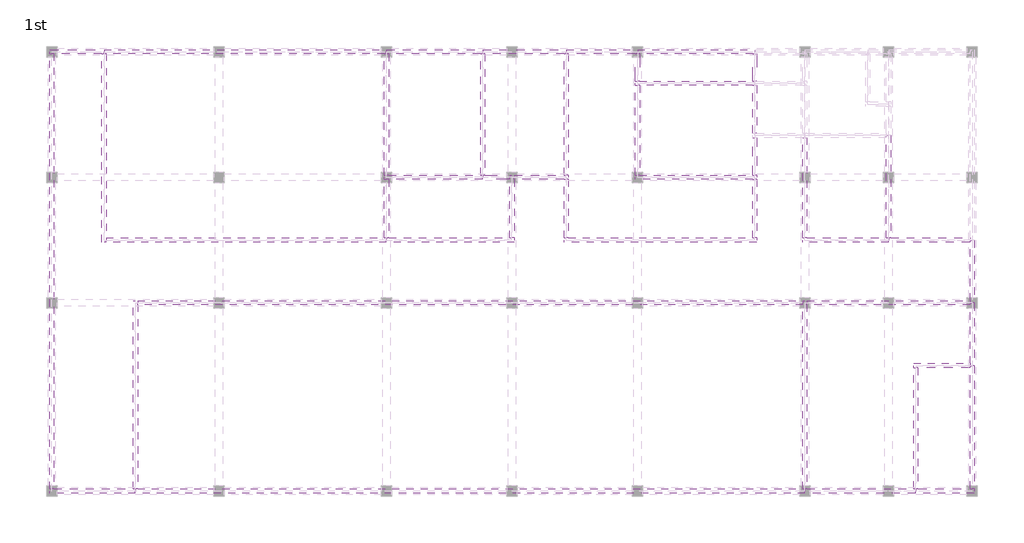
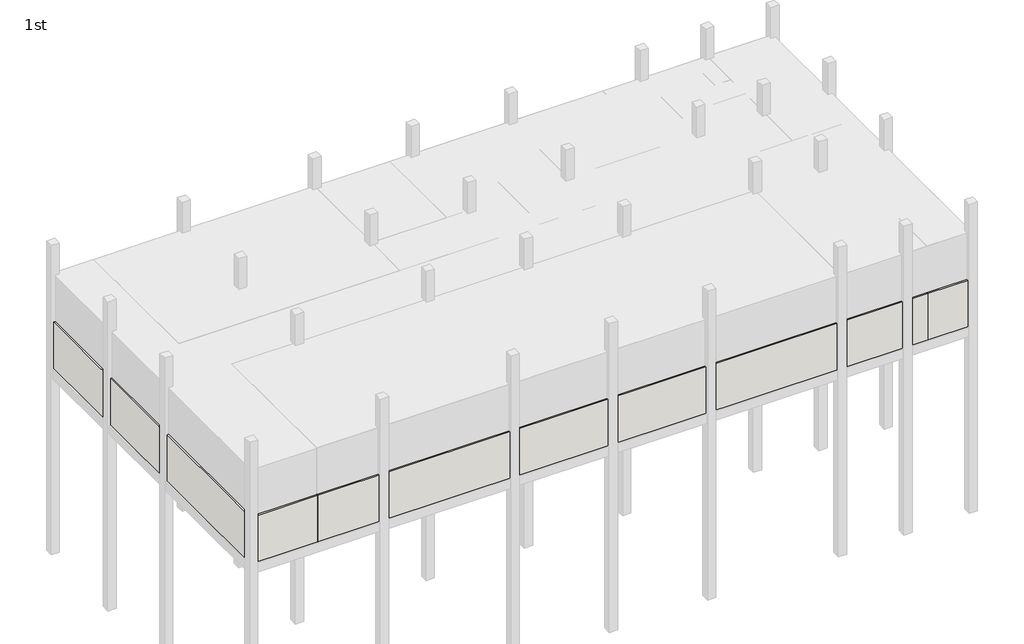
# One storey, part 1 of 3: 45 walls.
"""IFC4 building model written with IfcOpenShell, lengths in millimetres."""

from ifc_helpers import new_model, si_unit, frame, origin, place, context, project, spatial, polyline, outline, extrude, faceted_brep, element, save

model = new_model("IFC4")

# Units and contexts
model_context = context("Model", 3, world=origin())
ifc_project = project(units=[si_unit("LENGTHUNIT", "METRE", prefix="MILLI")], contexts=[model_context])

# Site, building, storey
site = spatial("IfcSite", under=ifc_project)
building = spatial("IfcBuilding", under=site)
storey = spatial("IfcBuildingStorey", under=building, Name="1st", Elevation=6000.0)

# Walls
placement = place(None, origin())
element("IfcWall", 1, ObjectType="WA111-Exterior RC Wall 200mm", at=placement, inside=storey, context=model_context, shape_type="Brep", body=[
    faceted_brep([(49459.6521483, 163823.8614395, 12000.0), (81459.6521483, 163823.8614395, 12000.0), (81459.6521483, 163823.8614395, 15000.0), (49459.6521483, 163823.8614395, 15000.0), (49459.6521483, 164023.8614395, 12000.0), (49459.6521483, 164023.8614395, 15000.0), (49559.6521483, 164023.8614395, 15000.0), (81359.6521483, 164023.8614395, 15000.0), (81459.6521483, 164023.8614395, 15000.0), (81459.6521483, 164023.8614395, 12000.0), (81359.6521483, 164023.8614395, 12000.0), (49559.6521483, 164023.8614395, 12000.0)], [[[0, 1, 2, 3]], [[4, 5, 6, 7, 8, 9, 10, 11]], [[1, 0, 4, 11, 10, 9]], [[2, 1, 9, 8]], [[3, 2, 8, 7, 6, 5]], [[0, 3, 5, 4]]]),
])
element("IfcWall", 2, ObjectType="WA111-Exterior RC Wall 200mm", at=placement, inside=storey, context=model_context, shape_type="Brep", body=[
    faceted_brep([(61459.6521483, 185023.8614395, 12000.0), (47959.6521483, 185023.8614395, 12000.0), (47959.6521483, 185023.8614395, 15000.0), (61459.6521483, 185023.8614395, 15000.0), (61459.6521483, 184823.8614395, 12000.0), (61459.6521483, 184823.8614395, 15000.0), (61359.6521483, 184823.8614395, 15000.0), (48059.6521483, 184823.8614395, 15000.0), (47959.6521483, 184823.8614395, 15000.0), (47959.6521483, 184823.8614395, 12000.0), (48059.6521483, 184823.8614395, 12000.0), (61359.6521483, 184823.8614395, 12000.0)], [[[0, 1, 2, 3]], [[4, 5, 6, 7, 8, 9, 10, 11]], [[1, 0, 4, 11, 10, 9]], [[2, 1, 9, 8]], [[3, 2, 8, 7, 6, 5]], [[0, 3, 5, 4]]]),
])
element("IfcWall", 3, ObjectType="WA111-Exterior RC Wall 200mm", at=placement, inside=storey, context=model_context, shape_type="Brep", body=[
    faceted_brep([(66059.6521483, 185023.8614395, 12000.0), (61459.6521483, 185023.8614395, 12000.0), (61459.6521483, 185023.8614395, 15000.0), (66059.6521483, 185023.8614395, 15000.0), (66059.6521483, 184823.8614395, 12000.0), (66059.6521483, 184823.8614395, 15000.0), (65959.6521483, 184823.8614395, 15000.0), (61559.6521483, 184823.8614395, 15000.0), (61459.6521483, 184823.8614395, 15000.0), (61459.6521483, 184823.8614395, 12000.0), (61559.6521483, 184823.8614395, 12000.0), (65959.6521483, 184823.8614395, 12000.0)], [[[0, 1, 2, 3]], [[4, 5, 6, 7, 8, 9, 10, 11]], [[1, 0, 4, 11, 10, 9]], [[2, 1, 9, 8]], [[3, 2, 8, 7, 6, 5]], [[0, 3, 5, 4]]]),
])
element("IfcWall", 4, ObjectType="WA111-Exterior RC Wall 200mm", at=placement, inside=storey, context=model_context, shape_type="Brep", body=[
    faceted_brep([(70059.6521483, 185023.8614395, 12000.0), (66059.6521483, 185023.8614395, 12000.0), (66059.6521483, 185023.8614395, 15000.0), (70059.6521483, 185023.8614395, 15000.0), (70059.6521483, 184823.8614395, 12000.0), (70059.6521483, 184823.8614395, 15000.0), (69959.6521483, 184823.8614395, 15000.0), (66159.6521483, 184823.8614395, 15000.0), (66059.6521483, 184823.8614395, 15000.0), (66059.6521483, 184823.8614395, 12000.0), (66159.6521483, 184823.8614395, 12000.0), (69959.6521483, 184823.8614395, 12000.0)], [[[0, 1, 2, 3]], [[4, 5, 6, 7, 8, 9, 10, 11]], [[1, 0, 4, 11, 10, 9]], [[2, 1, 9, 8]], [[3, 2, 8, 7, 6, 5]], [[0, 3, 5, 4]]]),
])
element("IfcWall", 5, ObjectType="WA111-Exterior RC Wall 200mm", at=placement, inside=storey, context=model_context, shape_type="Brep", body=[
    faceted_brep([(89559.6521483, 172923.8614395, 12000.0), (89559.6521483, 175923.8614395, 12000.0), (89559.6521483, 175923.8614395, 15000.0), (89559.6521483, 172923.8614395, 15000.0), (89359.6521483, 172923.8614395, 12000.0), (89359.6521483, 172923.8614395, 15000.0), (89359.6521483, 173023.8614395, 15000.0), (89359.6521483, 175823.8614395, 15000.0), (89359.6521483, 175923.8614395, 15000.0), (89359.6521483, 175923.8614395, 12000.0), (89359.6521483, 175823.8614395, 12000.0), (89359.6521483, 173023.8614395, 12000.0)], [[[0, 1, 2, 3]], [[4, 5, 6, 7, 8, 9, 10, 11]], [[1, 0, 4, 11, 10, 9]], [[2, 1, 9, 8]], [[3, 2, 8, 7, 6, 5]], [[0, 3, 5, 4]]]),
])
element("IfcWall", 6, ObjectType="WA111-Exterior RC Wall 200mm", at=placement, inside=storey, context=model_context, shape_type="Brep", body=[
    faceted_brep([(47959.6521483, 185023.8614395, 12000.0), (45359.6521483, 185023.8614395, 12000.0), (45359.6521483, 185023.8614395, 15000.0), (47959.6521483, 185023.8614395, 15000.0), (47959.6521483, 184823.8614395, 12000.0), (47959.6521483, 184823.8614395, 15000.0), (47859.6521483, 184823.8614395, 15000.0), (45559.6521483, 184823.8614395, 15000.0), (45359.6521483, 184823.8614395, 15000.0), (45359.6521483, 184823.8614395, 12000.0), (45559.6521483, 184823.8614395, 12000.0), (47859.6521483, 184823.8614395, 12000.0)], [[[0, 1, 2, 3]], [[4, 5, 6, 7, 8, 9, 10, 11]], [[1, 0, 4, 11, 10, 9]], [[3, 2, 8, 7, 6, 5]], [[0, 3, 5, 4]], [[2, 1, 9, 8]]]),
])
element("IfcWall", 7, ObjectType="WA111-Exterior RC Wall 200mm", at=placement, inside=storey, context=model_context, shape_type="SweptSolid", body=[
    extrude(outline(polyline([(45359.6521483, 164023.8614395), (45359.6521483, 184823.8614395), (45559.6521483, 184823.8614395), (45559.6521483, 164023.8614395), (45359.6521483, 164023.8614395)])), frame((0.0, 0.0, 12000.0), z_axis=(0.0, 0.0, 1.0), x_axis=(1.0, 0.0, 0.0)), (0.0, 0.0, 1.0), 3000.0),
])
element("IfcWall", 8, ObjectType="WA111-Exterior RC Wall 200mm", at=placement, inside=storey, context=model_context, shape_type="Brep", body=[
    faceted_brep([(45359.6521483, 163823.8614395, 12000.0), (49459.6521483, 163823.8614395, 12000.0), (49459.6521483, 163823.8614395, 15000.0), (45359.6521483, 163823.8614395, 15000.0), (45359.6521483, 164023.8614395, 12000.0), (45359.6521483, 164023.8614395, 15000.0), (45559.6521483, 164023.8614395, 15000.0), (49359.6521483, 164023.8614395, 15000.0), (49459.6521483, 164023.8614395, 15000.0), (49459.6521483, 164023.8614395, 12000.0), (49359.6521483, 164023.8614395, 12000.0), (45559.6521483, 164023.8614395, 12000.0)], [[[0, 1, 2, 3]], [[4, 5, 6, 7, 8, 9, 10, 11]], [[1, 0, 4, 11, 10, 9]], [[2, 1, 9, 8]], [[3, 2, 8, 7, 6, 5]], [[0, 3, 5, 4]]]),
])
element("IfcWall", 9, ObjectType="WA111-Exterior RC Wall 200mm", at=placement, inside=storey, context=model_context, shape_type="Brep", body=[
    faceted_brep([(79059.6521483, 185023.8614395, 12000.0), (73459.6521483, 185023.8614395, 12000.0), (73459.6521483, 185023.8614395, 15000.0), (79059.6521483, 185023.8614395, 15000.0), (79059.6521483, 184823.8614395, 12000.0), (79059.6521483, 184823.8614395, 15000.0), (78959.6521483, 184823.8614395, 15000.0), (73559.6521483, 184823.8614395, 15000.0), (73459.6521483, 184823.8614395, 15000.0), (73459.6521483, 184823.8614395, 12000.0), (73559.6521483, 184823.8614395, 12000.0), (78959.6521483, 184823.8614395, 12000.0)], [[[0, 1, 2, 3]], [[4, 5, 6, 7, 8, 9, 10, 11]], [[1, 0, 4, 11, 10, 9]], [[2, 1, 9, 8]], [[3, 2, 8, 7, 6, 5]], [[0, 3, 5, 4]]]),
])
element("IfcWall", 10, ObjectType="WA111-Exterior RC Wall 200mm", at=placement, inside=storey, context=model_context, shape_type="Brep", body=[
    faceted_brep([(73459.6521483, 185023.8614395, 12000.0), (70059.6521483, 185023.8614395, 12000.0), (70059.6521483, 185023.8614395, 15000.0), (73459.6521483, 185023.8614395, 15000.0), (73459.6521483, 184823.8614395, 12000.0), (73459.6521483, 184823.8614395, 15000.0), (73359.6521483, 184823.8614395, 15000.0), (70159.6521483, 184823.8614395, 15000.0), (70059.6521483, 184823.8614395, 15000.0), (70059.6521483, 184823.8614395, 12000.0), (70159.6521483, 184823.8614395, 12000.0), (73359.6521483, 184823.8614395, 12000.0)], [[[0, 1, 2, 3]], [[4, 5, 6, 7, 8, 9, 10, 11]], [[1, 0, 4, 11, 10, 9]], [[2, 1, 9, 8]], [[3, 2, 8, 7, 6, 5]], [[0, 3, 5, 4]]]),
])
element("IfcWall", 11, ObjectType="WA111-Exterior RC Wall 200mm", at=placement, inside=storey, context=model_context, shape_type="Brep", body=[
    faceted_brep([(81459.6521483, 163823.8614395, 12000.0), (86759.6521483, 163823.8614395, 12000.0), (86759.6521483, 163823.8614395, 15000.0), (81459.6521483, 163823.8614395, 15000.0), (81459.6521483, 164023.8614395, 12000.0), (81459.6521483, 164023.8614395, 15000.0), (81559.6521483, 164023.8614395, 15000.0), (86659.6521483, 164023.8614395, 15000.0), (86759.6521483, 164023.8614395, 15000.0), (86759.6521483, 164023.8614395, 12000.0), (86659.6521483, 164023.8614395, 12000.0), (81559.6521483, 164023.8614395, 12000.0)], [[[0, 1, 2, 3]], [[4, 5, 6, 7, 8, 9, 10, 11]], [[1, 0, 4, 11, 10, 9]], [[2, 1, 9, 8]], [[3, 2, 8, 7, 6, 5]], [[0, 3, 5, 4]]]),
])
element("IfcWall", 12, ObjectType="WA111-Exterior RC Wall 200mm", at=placement, inside=storey, context=model_context, shape_type="Brep", body=[
    faceted_brep([(89559.6521483, 169923.8614395, 12000.0), (89559.6521483, 172923.8614395, 12000.0), (89559.6521483, 172923.8614395, 15000.0), (89559.6521483, 169923.8614395, 15000.0), (89359.6521483, 169923.8614395, 12000.0), (89359.6521483, 169923.8614395, 15000.0), (89359.6521483, 170023.8614395, 15000.0), (89359.6521483, 172823.8614395, 15000.0), (89359.6521483, 172923.8614395, 15000.0), (89359.6521483, 172923.8614395, 12000.0), (89359.6521483, 172823.8614395, 12000.0), (89359.6521483, 170023.8614395, 12000.0)], [[[0, 1, 2, 3]], [[4, 5, 6, 7, 8, 9, 10, 11]], [[1, 0, 4, 11, 10, 9]], [[2, 1, 9, 8]], [[3, 2, 8, 7, 6, 5]], [[0, 3, 5, 4]]]),
])
element("IfcWall", 13, ObjectType="WA111-Exterior RC Wall 200mm", at=placement, inside=storey, context=model_context, shape_type="Brep", body=[
    faceted_brep([(89559.6521483, 164023.8614395, 12000.0), (89559.6521483, 169923.8614395, 12000.0), (89559.6521483, 169923.8614395, 15000.0), (89559.6521483, 164023.8614395, 15000.0), (89359.6521483, 164023.8614395, 12000.0), (89359.6521483, 164023.8614395, 15000.0), (89359.6521483, 169823.8614395, 15000.0), (89359.6521483, 169923.8614395, 15000.0), (89359.6521483, 169923.8614395, 12000.0), (89359.6521483, 169823.8614395, 12000.0)], [[[0, 1, 2, 3]], [[4, 5, 6, 7, 8, 9]], [[1, 0, 4, 9, 8]], [[2, 1, 8, 7]], [[3, 2, 7, 6, 5]], [[0, 3, 5, 4]]]),
])
element("IfcWall", 14, ObjectType="WA111-Exterior RC Wall 200mm", at=placement, inside=storey, context=model_context, shape_type="Brep", body=[
    faceted_brep([(86759.6521483, 163823.8614395, 12000.0), (89559.6521483, 163823.8614395, 12000.0), (89559.6521483, 163823.8614395, 15000.0), (86759.6521483, 163823.8614395, 15000.0), (86759.6521483, 164023.8614395, 12000.0), (86759.6521483, 164023.8614395, 15000.0), (86859.6521483, 164023.8614395, 15000.0), (89359.6521483, 164023.8614395, 15000.0), (89559.6521483, 164023.8614395, 15000.0), (89559.6521483, 164023.8614395, 12000.0), (89359.6521483, 164023.8614395, 12000.0), (86859.6521483, 164023.8614395, 12000.0)], [[[0, 1, 2, 3]], [[4, 5, 6, 7, 8, 9, 10, 11]], [[1, 0, 4, 11, 10, 9]], [[3, 2, 8, 7, 6, 5]], [[0, 3, 5, 4]], [[2, 1, 9, 8]]]),
])
element("IfcWall", 15, ObjectType="WA121-Interior RC Wall 200mm", at=placement, inside=storey, context=model_context, shape_type="SweptSolid", body=[
    extrude(outline(polyline([(49559.6521483, 173023.8614395), (81359.6521483, 173023.8614395), (81359.6521483, 172823.8614395), (49559.6521483, 172823.8614395), (49559.6521483, 173023.8614395)])), frame((0.0, 0.0, 12000.0), z_axis=(0.0, 0.0, 1.0), x_axis=(1.0, 0.0, 0.0)), (0.0, 0.0, 1.0), 3000.0),
])
element("IfcWall", 16, ObjectType="WA121-Interior RC Wall 200mm", at=placement, inside=storey, context=model_context, shape_type="Brep", body=[
    faceted_brep([(49359.6521483, 173023.8614395, 12000.0), (49359.6521483, 164023.8614395, 12000.0), (49359.6521483, 164023.8614395, 15000.0), (49359.6521483, 173023.8614395, 15000.0), (49559.6521483, 173023.8614395, 12000.0), (49559.6521483, 173023.8614395, 15000.0), (49559.6521483, 172823.8614395, 15000.0), (49559.6521483, 164023.8614395, 15000.0), (49559.6521483, 164023.8614395, 12000.0), (49559.6521483, 172823.8614395, 12000.0), (49459.6521483, 164023.8614395, 12000.0), (49459.6521483, 164023.8614395, 15000.0)], [[[0, 1, 2, 3]], [[4, 5, 6, 7, 8, 9]], [[1, 0, 4, 9, 8, 10]], [[3, 2, 11, 7, 6, 5]], [[0, 3, 5, 4]], [[2, 1, 10, 8, 7, 11]]]),
])
element("IfcWall", 17, ObjectType="WA121-Interior RC Wall 200mm", at=placement, inside=storey, context=model_context, shape_type="Brep", body=[
    faceted_brep([(81559.6521483, 164023.8614395, 12000.0), (81559.6521483, 172823.8614395, 12000.0), (81559.6521483, 173023.8614395, 12000.0), (81559.6521483, 173023.8614395, 15000.0), (81559.6521483, 172823.8614395, 15000.0), (81559.6521483, 164023.8614395, 15000.0), (81359.6521483, 164023.8614395, 12000.0), (81359.6521483, 164023.8614395, 15000.0), (81359.6521483, 172823.8614395, 15000.0), (81359.6521483, 173023.8614395, 15000.0), (81359.6521483, 173023.8614395, 12000.0), (81359.6521483, 172823.8614395, 12000.0), (81459.6521483, 164023.8614395, 12000.0), (81459.6521483, 164023.8614395, 15000.0)], [[[0, 1, 2, 3, 4, 5]], [[6, 7, 8, 9, 10, 11]], [[2, 1, 0, 12, 6, 11, 10]], [[5, 4, 3, 9, 8, 7, 13]], [[3, 2, 10, 9]], [[0, 5, 13, 7, 6, 12]]]),
])
element("IfcWall", 18, ObjectType="WA121-Interior RC Wall 200mm", at=placement, inside=storey, context=model_context, shape_type="Brep", body=[
    faceted_brep([(47859.6521483, 184823.8614395, 12000.0), (47859.6521483, 175823.8614395, 12000.0), (47859.6521483, 175823.8614395, 15000.0), (47859.6521483, 184823.8614395, 15000.0), (48059.6521483, 184823.8614395, 12000.0), (48059.6521483, 184823.8614395, 15000.0), (48059.6521483, 176023.8614395, 15000.0), (48059.6521483, 175823.8614395, 15000.0), (48059.6521483, 175823.8614395, 12000.0), (48059.6521483, 176023.8614395, 12000.0), (47959.6521483, 184823.8614395, 12000.0), (47959.6521483, 184823.8614395, 15000.0)], [[[0, 1, 2, 3]], [[4, 5, 6, 7, 8, 9]], [[1, 0, 10, 4, 9, 8]], [[3, 2, 7, 6, 5, 11]], [[0, 3, 11, 5, 4, 10]], [[2, 1, 8, 7]]]),
])
element("IfcWall", 19, ObjectType="WA121-Interior RC Wall 200mm", at=placement, inside=storey, context=model_context, shape_type="Brep", body=[
    faceted_brep([(48059.6521483, 175823.8614395, 12000.0), (61459.6521483, 175823.8614395, 12000.0), (61459.6521483, 175823.8614395, 15000.0), (48059.6521483, 175823.8614395, 15000.0), (48059.6521483, 176023.8614395, 12000.0), (48059.6521483, 176023.8614395, 15000.0), (61359.6521483, 176023.8614395, 15000.0), (61459.6521483, 176023.8614395, 15000.0), (61459.6521483, 176023.8614395, 12000.0), (61359.6521483, 176023.8614395, 12000.0)], [[[0, 1, 2, 3]], [[4, 5, 6, 7, 8, 9]], [[1, 0, 4, 9, 8]], [[2, 1, 8, 7]], [[3, 2, 7, 6, 5]], [[0, 3, 5, 4]]]),
])
element("IfcWall", 20, ObjectType="WA121-Interior RC Wall 200mm", at=placement, inside=storey, context=model_context, shape_type="Brep", body=[
    faceted_brep([(61559.6521483, 176023.8614395, 12000.0), (61559.6521483, 178823.8614395, 12000.0), (61559.6521483, 178823.8614395, 15000.0), (61559.6521483, 176023.8614395, 15000.0), (61359.6521483, 176023.8614395, 12000.0), (61359.6521483, 176023.8614395, 15000.0), (61359.6521483, 178823.8614395, 15000.0), (61359.6521483, 178823.8614395, 12000.0), (61459.6521483, 176023.8614395, 12000.0), (61459.6521483, 176023.8614395, 15000.0)], [[[0, 1, 2, 3]], [[4, 5, 6, 7]], [[1, 0, 8, 4, 7]], [[3, 2, 6, 5, 9]], [[0, 3, 9, 5, 4, 8]], [[2, 1, 7, 6]]]),
])
element("IfcWall", 21, ObjectType="WA121-Interior RC Wall 200mm", at=placement, inside=storey, context=model_context, shape_type="Brep", body=[
    faceted_brep([(61559.6521483, 179023.8614395, 12000.0), (61559.6521483, 184823.8614395, 12000.0), (61559.6521483, 184823.8614395, 15000.0), (61559.6521483, 179023.8614395, 15000.0), (61359.6521483, 179023.8614395, 12000.0), (61359.6521483, 179023.8614395, 15000.0), (61359.6521483, 184823.8614395, 15000.0), (61359.6521483, 184823.8614395, 12000.0), (61459.6521483, 184823.8614395, 12000.0), (61459.6521483, 184823.8614395, 15000.0)], [[[0, 1, 2, 3]], [[4, 5, 6, 7]], [[1, 0, 4, 7, 8]], [[3, 2, 9, 6, 5]], [[2, 1, 8, 7, 6, 9]], [[0, 3, 5, 4]]]),
])
element("IfcWall", 22, ObjectType="WA121-Interior RC Wall 200mm", at=placement, inside=storey, context=model_context, shape_type="Brep", body=[
    faceted_brep([(61359.6521483, 178823.8614395, 12000.0), (61559.6521483, 178823.8614395, 12000.0), (66059.6521483, 178823.8614395, 12000.0), (66059.6521483, 178823.8614395, 15000.0), (61559.6521483, 178823.8614395, 15000.0), (61359.6521483, 178823.8614395, 15000.0), (61359.6521483, 179023.8614395, 12000.0), (61359.6521483, 179023.8614395, 15000.0), (61559.6521483, 179023.8614395, 15000.0), (65959.6521483, 179023.8614395, 15000.0), (66059.6521483, 179023.8614395, 15000.0), (66059.6521483, 179023.8614395, 12000.0), (65959.6521483, 179023.8614395, 12000.0), (61559.6521483, 179023.8614395, 12000.0)], [[[0, 1, 2, 3, 4, 5]], [[6, 7, 8, 9, 10, 11, 12, 13]], [[2, 1, 0, 6, 13, 12, 11]], [[3, 2, 11, 10]], [[5, 4, 3, 10, 9, 8, 7]], [[0, 5, 7, 6]]]),
])
element("IfcWall", 23, ObjectType="WA121-Interior RC Wall 200mm", at=placement, inside=storey, context=model_context, shape_type="Brep", body=[
    faceted_brep([(66159.6521483, 179023.8614395, 12000.0), (66159.6521483, 184823.8614395, 12000.0), (66159.6521483, 184823.8614395, 15000.0), (66159.6521483, 179023.8614395, 15000.0), (65959.6521483, 179023.8614395, 12000.0), (65959.6521483, 179023.8614395, 15000.0), (65959.6521483, 184823.8614395, 15000.0), (65959.6521483, 184823.8614395, 12000.0), (66059.6521483, 179023.8614395, 12000.0), (66059.6521483, 184823.8614395, 12000.0), (66059.6521483, 184823.8614395, 15000.0), (66059.6521483, 179023.8614395, 15000.0)], [[[0, 1, 2, 3]], [[4, 5, 6, 7]], [[1, 0, 8, 4, 7, 9]], [[3, 2, 10, 6, 5, 11]], [[2, 1, 9, 7, 6, 10]], [[0, 3, 11, 5, 4, 8]]]),
])
element("IfcWall", 24, ObjectType="WA121-Interior RC Wall 200mm", at=placement, inside=storey, context=model_context, shape_type="Brep", body=[
    faceted_brep([(81359.6521483, 180823.8614395, 12000.0), (81359.6521483, 176023.8614395, 12000.0), (81359.6521483, 176023.8614395, 15000.0), (81359.6521483, 180823.8614395, 15000.0), (81559.6521483, 180823.8614395, 12000.0), (81559.6521483, 180823.8614395, 15000.0), (81559.6521483, 176023.8614395, 15000.0), (81559.6521483, 176023.8614395, 12000.0), (81459.6521483, 180823.8614395, 12000.0), (81459.6521483, 180823.8614395, 15000.0)], [[[0, 1, 2, 3]], [[4, 5, 6, 7]], [[1, 0, 8, 4, 7]], [[3, 2, 6, 5, 9]], [[0, 3, 9, 5, 4, 8]], [[2, 1, 7, 6]]]),
])
element("IfcWall", 25, ObjectType="WA121-Interior RC Wall 200mm", at=placement, inside=storey, context=model_context, shape_type="Brep", body=[
    faceted_brep([(81359.6521483, 175823.8614395, 12000.0), (85459.6521483, 175823.8614395, 12000.0), (85459.6521483, 175823.8614395, 15000.0), (81359.6521483, 175823.8614395, 15000.0), (81359.6521483, 176023.8614395, 12000.0), (81359.6521483, 176023.8614395, 15000.0), (81559.6521483, 176023.8614395, 15000.0), (85359.6521483, 176023.8614395, 15000.0), (85459.6521483, 176023.8614395, 15000.0), (85459.6521483, 176023.8614395, 12000.0), (85359.6521483, 176023.8614395, 12000.0), (81559.6521483, 176023.8614395, 12000.0)], [[[0, 1, 2, 3]], [[4, 5, 6, 7, 8, 9, 10, 11]], [[1, 0, 4, 11, 10, 9]], [[2, 1, 9, 8]], [[3, 2, 8, 7, 6, 5]], [[0, 3, 5, 4]]]),
])
element("IfcWall", 26, ObjectType="WA121-Interior RC Wall 200mm", at=placement, inside=storey, context=model_context, shape_type="Brep", body=[
    faceted_brep([(85559.6521483, 176023.8614395, 12000.0), (85559.6521483, 180923.8614395, 12000.0), (85559.6521483, 180923.8614395, 15000.0), (85559.6521483, 176023.8614395, 15000.0), (85359.6521483, 176023.8614395, 12000.0), (85359.6521483, 176023.8614395, 15000.0), (85359.6521483, 180823.8614395, 15000.0), (85359.6521483, 180923.8614395, 15000.0), (85359.6521483, 180923.8614395, 12000.0), (85359.6521483, 180823.8614395, 12000.0), (85459.6521483, 176023.8614395, 12000.0), (85459.6521483, 176023.8614395, 15000.0)], [[[0, 1, 2, 3]], [[4, 5, 6, 7, 8, 9]], [[1, 0, 10, 4, 9, 8]], [[2, 1, 8, 7]], [[3, 2, 7, 6, 5, 11]], [[0, 3, 11, 5, 4, 10]]]),
])
element("IfcWall", 27, ObjectType="WA121-Interior RC Wall 200mm", at=placement, inside=storey, context=model_context, shape_type="Brep", body=[
    faceted_brep([(85459.6521483, 175823.8614395, 12000.0), (89359.6521483, 175823.8614395, 12000.0), (89359.6521483, 175823.8614395, 15000.0), (85459.6521483, 175823.8614395, 15000.0), (85459.6521483, 176023.8614395, 12000.0), (85459.6521483, 176023.8614395, 15000.0), (85559.6521483, 176023.8614395, 15000.0), (89359.6521483, 176023.8614395, 15000.0), (89359.6521483, 176023.8614395, 12000.0), (85559.6521483, 176023.8614395, 12000.0), (89359.6521483, 175923.8614395, 12000.0), (89359.6521483, 175923.8614395, 15000.0)], [[[0, 1, 2, 3]], [[4, 5, 6, 7, 8, 9]], [[1, 0, 4, 9, 8, 10]], [[3, 2, 11, 7, 6, 5]], [[0, 3, 5, 4]], [[2, 1, 10, 8, 7, 11]]]),
])
element("IfcWall", 28, ObjectType="WA121-Interior RC Wall 200mm", at=placement, inside=storey, context=model_context, shape_type="Brep", body=[
    faceted_brep([(66059.6521483, 178823.8614395, 12000.0), (67359.6521483, 178823.8614395, 12000.0), (67359.6521483, 178823.8614395, 15000.0), (66059.6521483, 178823.8614395, 15000.0), (66059.6521483, 179023.8614395, 12000.0), (66059.6521483, 179023.8614395, 15000.0), (66159.6521483, 179023.8614395, 15000.0), (67359.6521483, 179023.8614395, 15000.0), (67359.6521483, 179023.8614395, 12000.0), (66159.6521483, 179023.8614395, 12000.0)], [[[0, 1, 2, 3]], [[4, 5, 6, 7, 8, 9]], [[1, 0, 4, 9, 8]], [[3, 2, 7, 6, 5]], [[0, 3, 5, 4]], [[2, 1, 8, 7]]]),
])
element("IfcWall", 29, ObjectType="WA121-Interior RC Wall 200mm", at=placement, inside=storey, context=model_context, shape_type="Brep", body=[
    faceted_brep([(67559.6521483, 178823.8614395, 12000.0), (69959.6521483, 178823.8614395, 12000.0), (70159.6521483, 178823.8614395, 12000.0), (70159.6521483, 178823.8614395, 15000.0), (69959.6521483, 178823.8614395, 15000.0), (67559.6521483, 178823.8614395, 15000.0), (67559.6521483, 179023.8614395, 12000.0), (67559.6521483, 179023.8614395, 15000.0), (69959.6521483, 179023.8614395, 15000.0), (70159.6521483, 179023.8614395, 15000.0), (70159.6521483, 179023.8614395, 12000.0), (69959.6521483, 179023.8614395, 12000.0)], [[[0, 1, 2, 3, 4, 5]], [[6, 7, 8, 9, 10, 11]], [[2, 1, 0, 6, 11, 10]], [[5, 4, 3, 9, 8, 7]], [[3, 2, 10, 9]], [[0, 5, 7, 6]]]),
])
element("IfcWall", 30, ObjectType="WA121-Interior RC Wall 200mm", at=placement, inside=storey, context=model_context, shape_type="Brep", body=[
    faceted_brep([(70159.6521483, 179023.8614395, 12000.0), (70159.6521483, 184823.8614395, 12000.0), (70159.6521483, 184823.8614395, 15000.0), (70159.6521483, 179023.8614395, 15000.0), (69959.6521483, 179023.8614395, 12000.0), (69959.6521483, 179023.8614395, 15000.0), (69959.6521483, 184823.8614395, 15000.0), (69959.6521483, 184823.8614395, 12000.0), (70059.6521483, 184823.8614395, 12000.0), (70059.6521483, 184823.8614395, 15000.0)], [[[0, 1, 2, 3]], [[4, 5, 6, 7]], [[1, 0, 4, 7, 8]], [[3, 2, 9, 6, 5]], [[2, 1, 8, 7, 6, 9]], [[0, 3, 5, 4]]]),
])
element("IfcWall", 31, ObjectType="WA121-Interior RC Wall 200mm", at=placement, inside=storey, context=model_context, shape_type="Brep", body=[
    faceted_brep([(61459.6521483, 175823.8614395, 12000.0), (67559.6521483, 175823.8614395, 12000.0), (67559.6521483, 175823.8614395, 15000.0), (61459.6521483, 175823.8614395, 15000.0), (61459.6521483, 176023.8614395, 12000.0), (61459.6521483, 176023.8614395, 15000.0), (61559.6521483, 176023.8614395, 15000.0), (67359.6521483, 176023.8614395, 15000.0), (67559.6521483, 176023.8614395, 15000.0), (67559.6521483, 176023.8614395, 12000.0), (67359.6521483, 176023.8614395, 12000.0), (61559.6521483, 176023.8614395, 12000.0)], [[[0, 1, 2, 3]], [[4, 5, 6, 7, 8, 9, 10, 11]], [[1, 0, 4, 11, 10, 9]], [[3, 2, 8, 7, 6, 5]], [[0, 3, 5, 4]], [[2, 1, 9, 8]]]),
])
element("IfcWall", 32, ObjectType="WA121-Interior RC Wall 200mm", at=placement, inside=storey, context=model_context, shape_type="Brep", body=[
    faceted_brep([(67559.6521483, 176023.8614395, 12000.0), (67559.6521483, 178823.8614395, 12000.0), (67559.6521483, 179023.8614395, 12000.0), (67559.6521483, 179023.8614395, 15000.0), (67559.6521483, 178823.8614395, 15000.0), (67559.6521483, 176023.8614395, 15000.0), (67359.6521483, 176023.8614395, 12000.0), (67359.6521483, 176023.8614395, 15000.0), (67359.6521483, 178823.8614395, 15000.0), (67359.6521483, 179023.8614395, 15000.0), (67359.6521483, 179023.8614395, 12000.0), (67359.6521483, 178823.8614395, 12000.0)], [[[0, 1, 2, 3, 4, 5]], [[6, 7, 8, 9, 10, 11]], [[2, 1, 0, 6, 11, 10]], [[5, 4, 3, 9, 8, 7]], [[3, 2, 10, 9]], [[0, 5, 7, 6]]]),
])
element("IfcWall", 33, ObjectType="WA121-Interior RC Wall 200mm", at=placement, inside=storey, context=model_context, shape_type="Brep", body=[
    faceted_brep([(78959.6521483, 184823.8614395, 12000.0), (78959.6521483, 183523.8614395, 12000.0), (78959.6521483, 183523.8614395, 15000.0), (78959.6521483, 184823.8614395, 15000.0), (79159.6521483, 184823.8614395, 12000.0), (79159.6521483, 184823.8614395, 15000.0), (79159.6521483, 183523.8614395, 15000.0), (79159.6521483, 183523.8614395, 12000.0), (79059.6521483, 184823.8614395, 12000.0), (79059.6521483, 183523.8614395, 12000.0), (79059.6521483, 183523.8614395, 15000.0), (79059.6521483, 184823.8614395, 15000.0)], [[[0, 1, 2, 3]], [[4, 5, 6, 7]], [[1, 0, 8, 4, 7, 9]], [[3, 2, 10, 6, 5, 11]], [[0, 3, 11, 5, 4, 8]], [[2, 1, 9, 7, 6, 10]]]),
])
element("IfcWall", 34, ObjectType="WA121-Interior RC Wall 200mm", at=placement, inside=storey, context=model_context, shape_type="Brep", body=[
    faceted_brep([(81559.6521483, 172823.8614395, 12000.0), (89359.6521483, 172823.8614395, 12000.0), (89359.6521483, 172823.8614395, 15000.0), (81559.6521483, 172823.8614395, 15000.0), (81559.6521483, 173023.8614395, 12000.0), (81559.6521483, 173023.8614395, 15000.0), (89359.6521483, 173023.8614395, 15000.0), (89359.6521483, 173023.8614395, 12000.0), (89359.6521483, 172923.8614395, 12000.0), (89359.6521483, 172923.8614395, 15000.0)], [[[0, 1, 2, 3]], [[4, 5, 6, 7]], [[1, 0, 4, 7, 8]], [[3, 2, 9, 6, 5]], [[0, 3, 5, 4]], [[2, 1, 8, 7, 6, 9]]]),
])
element("IfcWall", 35, ObjectType="WA121-Interior RC Wall 200mm", at=placement, inside=storey, context=model_context, shape_type="SweptSolid", body=[
    extrude(outline(polyline([(78959.6521483, 179023.8614395), (78959.6521483, 180823.8614395), (79159.6521483, 180823.8614395), (79159.6521483, 179023.8614395), (78959.6521483, 179023.8614395)])), frame((0.0, 0.0, 12000.0), z_axis=(0.0, 0.0, 1.0), x_axis=(1.0, 0.0, 0.0)), (0.0, 0.0, 1.0), 3000.0),
])
element("IfcWall", 36, ObjectType="WA121-Interior RC Wall 200mm", at=placement, inside=storey, context=model_context, shape_type="SweptSolid", body=[
    extrude(outline(polyline([(78959.6521483, 176023.8614395), (78959.6521483, 178823.8614395), (79159.6521483, 178823.8614395), (79159.6521483, 176023.8614395), (78959.6521483, 176023.8614395)])), frame((0.0, 0.0, 12000.0), z_axis=(0.0, 0.0, 1.0), x_axis=(1.0, 0.0, 0.0)), (0.0, 0.0, 1.0), 3000.0),
])
element("IfcWall", 37, ObjectType="WA121-Interior RC Wall 200mm", at=placement, inside=storey, context=model_context, shape_type="Brep", body=[
    faceted_brep([(79159.6521483, 176023.8614395, 12000.0), (78959.6521483, 176023.8614395, 12000.0), (70159.6521483, 176023.8614395, 12000.0), (69959.6521483, 176023.8614395, 12000.0), (69959.6521483, 176023.8614395, 15000.0), (70159.6521483, 176023.8614395, 15000.0), (78959.6521483, 176023.8614395, 15000.0), (79159.6521483, 176023.8614395, 15000.0), (79159.6521483, 175823.8614395, 12000.0), (79159.6521483, 175823.8614395, 15000.0), (69959.6521483, 175823.8614395, 15000.0), (69959.6521483, 175823.8614395, 12000.0)], [[[0, 1, 2, 3, 4, 5, 6, 7]], [[8, 9, 10, 11]], [[3, 2, 1, 0, 8, 11]], [[7, 6, 5, 4, 10, 9]], [[0, 7, 9, 8]], [[4, 3, 11, 10]]]),
])
element("IfcWall", 38, ObjectType="WA121-Interior RC Wall 200mm", at=placement, inside=storey, context=model_context, shape_type="SweptSolid", body=[
    extrude(outline(polyline([(70159.6521483, 178823.8614395), (70159.6521483, 176023.8614395), (69959.6521483, 176023.8614395), (69959.6521483, 178823.8614395), (70159.6521483, 178823.8614395)])), frame((0.0, 0.0, 12000.0), z_axis=(0.0, 0.0, 1.0), x_axis=(1.0, 0.0, 0.0)), (0.0, 0.0, 1.0), 3000.0),
])
element("IfcWall", 39, ObjectType="WA121-Interior RC Wall 200mm", at=placement, inside=storey, context=model_context, shape_type="Brep", body=[
    faceted_brep([(78959.6521483, 183323.8614395, 12000.0), (78959.6521483, 181023.8614395, 12000.0), (78959.6521483, 181023.8614395, 15000.0), (78959.6521483, 183323.8614395, 15000.0), (79159.6521483, 183323.8614395, 12000.0), (79159.6521483, 183323.8614395, 15000.0), (79159.6521483, 181023.8614395, 15000.0), (79159.6521483, 181023.8614395, 12000.0), (79059.6521483, 183323.8614395, 12000.0), (79059.6521483, 183323.8614395, 15000.0)], [[[0, 1, 2, 3]], [[4, 5, 6, 7]], [[1, 0, 8, 4, 7]], [[3, 2, 6, 5, 9]], [[0, 3, 9, 5, 4, 8]], [[2, 1, 7, 6]]]),
])
element("IfcWall", 40, ObjectType="WA121-Interior RC Wall 200mm", at=placement, inside=storey, context=model_context, shape_type="Brep", body=[
    faceted_brep([(73359.6521483, 184823.8614395, 12000.0), (73359.6521483, 183523.8614395, 12000.0), (73359.6521483, 183523.8614395, 15000.0), (73359.6521483, 184823.8614395, 15000.0), (73559.6521483, 184823.8614395, 12000.0), (73559.6521483, 184823.8614395, 15000.0), (73559.6521483, 183523.8614395, 15000.0), (73559.6521483, 183523.8614395, 12000.0), (73459.6521483, 184823.8614395, 12000.0), (73459.6521483, 184823.8614395, 15000.0)], [[[0, 1, 2, 3]], [[4, 5, 6, 7]], [[1, 0, 8, 4, 7]], [[3, 2, 6, 5, 9]], [[0, 3, 9, 5, 4, 8]], [[2, 1, 7, 6]]]),
])
element("IfcWall", 41, ObjectType="WA121-Interior RC Wall 200mm", at=placement, inside=storey, context=model_context, shape_type="Brep", body=[
    faceted_brep([(73359.6521483, 183323.8614395, 12000.0), (73559.6521483, 183323.8614395, 12000.0), (78959.6521483, 183323.8614395, 12000.0), (79059.6521483, 183323.8614395, 12000.0), (79059.6521483, 183323.8614395, 15000.0), (78959.6521483, 183323.8614395, 15000.0), (73559.6521483, 183323.8614395, 15000.0), (73359.6521483, 183323.8614395, 15000.0), (73359.6521483, 183523.8614395, 12000.0), (73359.6521483, 183523.8614395, 15000.0), (73559.6521483, 183523.8614395, 15000.0), (78959.6521483, 183523.8614395, 15000.0), (79059.6521483, 183523.8614395, 15000.0), (79059.6521483, 183523.8614395, 12000.0), (78959.6521483, 183523.8614395, 12000.0), (73559.6521483, 183523.8614395, 12000.0)], [[[0, 1, 2, 3, 4, 5, 6, 7]], [[8, 9, 10, 11, 12, 13, 14, 15]], [[3, 2, 1, 0, 8, 15, 14, 13]], [[4, 3, 13, 12]], [[7, 6, 5, 4, 12, 11, 10, 9]], [[0, 7, 9, 8]]]),
])
element("IfcWall", 42, ObjectType="WA121-Interior RC Wall 200mm", at=placement, inside=storey, context=model_context, shape_type="Brep", body=[
    faceted_brep([(79159.6521483, 179023.8614395, 12000.0), (78959.6521483, 179023.8614395, 12000.0), (73559.6521483, 179023.8614395, 12000.0), (73359.6521483, 179023.8614395, 12000.0), (73359.6521483, 179023.8614395, 15000.0), (73559.6521483, 179023.8614395, 15000.0), (78959.6521483, 179023.8614395, 15000.0), (79159.6521483, 179023.8614395, 15000.0), (79159.6521483, 178823.8614395, 12000.0), (79159.6521483, 178823.8614395, 15000.0), (78959.6521483, 178823.8614395, 15000.0), (73359.6521483, 178823.8614395, 15000.0), (73359.6521483, 178823.8614395, 12000.0), (78959.6521483, 178823.8614395, 12000.0)], [[[0, 1, 2, 3, 4, 5, 6, 7]], [[8, 9, 10, 11, 12, 13]], [[3, 2, 1, 0, 8, 13, 12]], [[7, 6, 5, 4, 11, 10, 9]], [[0, 7, 9, 8]], [[4, 3, 12, 11]]]),
])
element("IfcWall", 43, ObjectType="WA121-Interior RC Wall 200mm", at=placement, inside=storey, context=model_context, shape_type="SweptSolid", body=[
    extrude(outline(polyline([(73559.6521483, 183323.8614395), (73559.6521483, 179023.8614395), (73359.6521483, 179023.8614395), (73359.6521483, 183323.8614395), (73559.6521483, 183323.8614395)])), frame((0.0, 0.0, 12000.0), z_axis=(0.0, 0.0, 1.0), x_axis=(1.0, 0.0, 0.0)), (0.0, 0.0, 1.0), 3000.0),
])
element("IfcWall", 44, ObjectType="WA121-Interior RC Wall 200mm", at=placement, inside=storey, context=model_context, shape_type="Brep", body=[
    faceted_brep([(86859.6521483, 164023.8614395, 12000.0), (86859.6521483, 169823.8614395, 12000.0), (86859.6521483, 169823.8614395, 15000.0), (86859.6521483, 164023.8614395, 15000.0), (86659.6521483, 164023.8614395, 12000.0), (86659.6521483, 164023.8614395, 15000.0), (86659.6521483, 169823.8614395, 15000.0), (86659.6521483, 169823.8614395, 12000.0), (86759.6521483, 164023.8614395, 12000.0), (86759.6521483, 164023.8614395, 15000.0)], [[[0, 1, 2, 3]], [[4, 5, 6, 7]], [[1, 0, 8, 4, 7]], [[3, 2, 6, 5, 9]], [[2, 1, 7, 6]], [[0, 3, 9, 5, 4, 8]]]),
])
element("IfcWall", 45, ObjectType="WA121-Interior RC Wall 200mm", at=placement, inside=storey, context=model_context, shape_type="Brep", body=[
    faceted_brep([(86659.6521483, 169823.8614395, 12000.0), (86859.6521483, 169823.8614395, 12000.0), (89359.6521483, 169823.8614395, 12000.0), (89359.6521483, 169823.8614395, 15000.0), (86859.6521483, 169823.8614395, 15000.0), (86659.6521483, 169823.8614395, 15000.0), (86659.6521483, 170023.8614395, 12000.0), (86659.6521483, 170023.8614395, 15000.0), (89359.6521483, 170023.8614395, 15000.0), (89359.6521483, 170023.8614395, 12000.0), (89359.6521483, 169923.8614395, 12000.0), (89359.6521483, 169923.8614395, 15000.0)], [[[0, 1, 2, 3, 4, 5]], [[6, 7, 8, 9]], [[2, 1, 0, 6, 9, 10]], [[5, 4, 3, 11, 8, 7]], [[0, 5, 7, 6]], [[3, 2, 10, 9, 8, 11]]]),
])

save(model, "model.ifc")

# Revit data of these elements
# Type "WA111-Exterior RC Wall 200mm"
#   Type Comments = ""
#   Layers, outside or top first: 0 mm "A04AL077-00001_Ext Wall Painting_Acrylic Emulsion Paint" (function 100); 200 mm "A03AD032-00007_Structural Concrete_25MPa-30MPa" (function 1); 0 mm "A03AD036-00001_Form Work (1 time in use)" (function 100); 0 mm "A04AL078-00002_Int Wall Painting_Water Emulsion Paint" (function 100); 0 mm "A04AL081-00001_Skirt_Acrylic Emulsion Paint" (function 100)
# Type "WA121-Interior RC Wall 200mm"
#   Type Comments = ""
#   Layers, outside or top first: 0 mm "A04AL081-00001_Skirt_Acrylic Emulsion Paint" (function 100); 0 mm "A04AL078-00002_Int Wall Painting_Water Emulsion Paint" (function 100); 200 mm "A03AD032-00007_Structural Concrete_25MPa-30MPa" (function 1); 0 mm "A03AD036-00001_Form Work (1 time in use)" (function 100); 0 mm "A04AL078-00002_Int Wall Painting_Water Emulsion Paint" (function 100); 0 mm "A04AL081-00001_Skirt_Acrylic Emulsion Paint" (function 100)
# Elements 1, 2, 3, 4, 5, 7, 9, 10, 11, 12, 13 (IfcWall, "WA111-Exterior RC Wall 200mm")
#   Top Offset = -1200 mm
#   Base Offset = 0 mm
#   Unconnected Height = 3000 mm
#   wall height = 3000 mm
#   Phase Created = New Construction
#   Base Constraint = 2nd
#   Materials on its faces: "Default Wall", "A03AD032-00007_Structural Concrete_25MPa-30MPa"
# Elements 6, 8, 14 (IfcWall, "WA111-Exterior RC Wall 200mm")
#   Top Offset = -1200 mm
#   Base Offset = 0 mm
#   Unconnected Height = 3000 mm
#   wall height = 3000 mm
#   Phase Created = New Construction
#   Base Constraint = 2nd
#   Materials on its faces: "A03AD032-00007_Structural Concrete_25MPa-30MPa", "Default Wall"
# Elements 15, 19, 20, 21, 23, 24, 26, 27, 28, 30, 33, 34, 35, 36, 38, 39, 40, 43, 44 (IfcWall, "WA121-Interior RC Wall 200mm")
#   Top Offset = 0 mm
#   Base Offset = 0 mm
#   Unconnected Height = 3000 mm
#   wall height = 3000 mm
#   Phase Created = New Construction
#   Base Constraint = 2nd
#   Materials on its faces: "Default Wall", "A03AD032-00007_Structural Concrete_25MPa-30MPa"
# Elements 16, 17, 18, 22, 25, 29, 31, 32, 37, 41, 42, 45 (IfcWall, "WA121-Interior RC Wall 200mm")
#   Top Offset = 0 mm
#   Base Offset = 0 mm
#   Unconnected Height = 3000 mm
#   wall height = 3000 mm
#   Phase Created = New Construction
#   Base Constraint = 2nd
#   Materials on its faces: "A03AD032-00007_Structural Concrete_25MPa-30MPa", "Default Wall"
# Materials
#   "A04AL077-00001_Ext Wall Painting_Acrylic Emulsion Paint": class "Finish", colour RGB 128 128 64, transparency 0, Description = "Plastic", W00) Work Master Code = "A04AL077-00001", W01) Work Master_Lv1 = "Finishing Work", W02) Work Master_Lv2 = "Painting Work", W03) Work Master_Spec.1 = "External Wall Painting", W04) Work Master_Spec.2 = "Acrylic Emulsion Paint", Cost = 0
#   "A03AD032-00007_Structural Concrete_25MPa-30MPa": class "Concrete", colour RGB 176 176 176, transparency 0, Keynote = "09910.A1", Description = "LATEX PAINT ON F.F CONC.", W00) Work Master Code = "A03AD032-00007", W01) Work Master_Lv1 = "Concrete Work", W02) Work Master_Lv2 = "Superstructure Work", W03) Work Master_Spec.1 = "Structural Concrete", W04) Work Master_Spec.2 = "Cement Type-1", W05) Work Master_Spec.3 = "25MPa < F'c (Cylinder Strength) ≤ 30MPa", Cost = 0
#   "A03AD036-00001_Form Work (1 time in use)": class "Wood", colour RGB 149 120 74, transparency 0, Description = "Plywood", W00) Work Master Code = "A03AD036-00001", W01) Work Master_Lv1 = "Concrete Work", W02) Work Master_Lv2 = "Superstructure Work", W03) Work Master_Spec.1 = "Form Work (1 time in use)", W04) Work Master_Spec.2 = "Flat Form", W05) Work Master_Spec.3 = "Dressed Lumber, Plywood or Steel Form(Wood Planks are not Allowed) incl. Chamfer", Cost = 0
#   "A04AL078-00002_Int Wall Painting_Water Emulsion Paint": class "Finish", colour RGB 128 128 64, transparency 0, Description = "Plastic", W00) Work Master Code = "A04AL078-00002", W01) Work Master_Lv1 = "Finishing Work", W02) Work Master_Lv2 = "Painting Work", W03) Work Master_Spec.1 = "Internal Wall Painting", W04) Work Master_Spec.2 = "Water Emulsion Paint", Cost = 0
#   "A04AL081-00001_Skirt_Acrylic Emulsion Paint": class "Finish", colour RGB 128 128 64, transparency 0, Description = "Plastic", W00) Work Master Code = "A04AL081-00001", W01) Work Master_Lv1 = "Finishing Work", W02) Work Master_Lv2 = "Painting Work", W03) Work Master_Spec.1 = "Skirt Painting", W04) Work Master_Spec.2 = "Acrylic Emulsion Paint", W05) Work Master_Spec.3 = "100mm≤H<150mm", Cost = 0
#   "Default Wall": class "Miscellaneous", colour RGB 80 80 80, transparency 0
# Room at (65459.652, 168423.861) mm, phase "New Construction", upper offset 2438.4 mm, lower offset 0 mm
#   Department = "CI"
#   Number = "3.0"
#   Name = "Central Control Room"
#   Interior Finish = "IF3"
#   Exterior Finish = "EF1"
# Room at (54709.652, 180423.861) mm, phase "New Construction", upper offset 2438.4 mm, lower offset 0 mm
#   Department = "CI"
#   Number = "3.1"
#   Name = "Engineer Room"
#   Interior Finish = "IF3"
#   Exterior Finish = "EF1"
# Room at (63759.652, 181923.861) mm, phase "New Construction", upper offset 2438.4 mm, lower offset 0 mm
#   Department = "AR"
#   Number = "3.2"
#   Name = "Document Room"
#   Interior Finish = "IF2-1"
#   Exterior Finish = "EF1"
# Room at (83459.652, 178423.861) mm, phase "New Construction", upper offset 2438.4 mm, lower offset 0 mm
#   Department = "AR"
#   Number = "3.3"
#   Name = "Toilet (M)"
#   Interior Finish = "IF5"
#   Exterior Finish = "EF1"
# Room at (87459.652, 180423.861) mm, phase "New Construction", upper offset 2438.4 mm, lower offset 0 mm
#   Department = "AR"
#   Number = "3.4"
#   Name = "Stairway"
#   Interior Finish = "IF2"
#   Exterior Finish = "EF1"
# Room at (68059.652, 181923.861) mm, phase "New Construction", upper offset 2438.4 mm, lower offset 0 mm
#   Department = "AR"
#   Number = "3.5"
#   Name = "Shift Office Room"
#   Interior Finish = "IF2-1"
#   Exterior Finish = "EF1"
# Room at (64459.652, 177423.861) mm, phase "New Construction", upper offset 2438.4 mm, lower offset 0 mm
#   Department = "AR"
#   Number = "3.6"
#   Name = "LOTO Office Room"
#   Interior Finish = "IF2-1"
#   Exterior Finish = "EF1"
# Room at (80259.652, 184173.861) mm, phase "New Construction", upper offset 2438.4 mm, lower offset 0 mm
#   Department = "AR"
#   Number = "3.7"
#   Name = "Shower Room (F)"
#   Interior Finish = "IF5"
#   Exterior Finish = "EF1"
# Room at (67459.652, 174423.861) mm, phase "New Construction", upper offset 2438.4 mm, lower offset 0 mm
#   Department = "AR"
#   Number = "3.8"
#   Name = "Corridor"
#   Interior Finish = "IF2-1"
#   Exterior Finish = "EF1"
# Room at (80259.652, 182173.861) mm, phase "New Construction", upper offset 2438.4 mm, lower offset 0 mm
#   Department = "AR"
#   Number = "3.9"
#   Name = "Locker Room (F)"
#   Interior Finish = "IF2-1"
#   Exterior Finish = "EF1"
# Room at (76259.652, 184173.861) mm, phase "New Construction", upper offset 2438.4 mm, lower offset 0 mm
#   Department = "AR"
#   Number = "3.10"
#   Name = "Shower Room (M)"
#   Interior Finish = "IF5"
#   Exterior Finish = "EF1"
# Room at (74559.652, 178751.292) mm, phase "New Construction", upper offset 2438.4 mm, lower offset 0 mm
#   Department = "AR"
#   Number = "3.11"
#   Name = "Kitch & Lunch Room"
#   Interior Finish = "IF2-1"
#   Exterior Finish = "EF1"
# Room at (76259.652, 181173.861) mm, phase "New Construction", upper offset 2438.4 mm, lower offset 0 mm
#   Department = "AR"
#   Number = "3.12"
#   Name = "Locker Room (M)"
#   Interior Finish = "IF2-1"
#   Exterior Finish = "EF1"
# Room at (85459.652, 168423.861) mm, phase "New Construction", upper offset 2438.4 mm, lower offset 0 mm
#   Department = "SF"
#   Number = "3.13"
#   Name = "Fire Gas Room"
#   Interior Finish = "IF1"
#   Exterior Finish = "EF1"
# Room at (88109.652, 166923.861) mm, phase "New Construction", upper offset 2438.4 mm, lower offset 0 mm
#   Department = "HV"
#   Number = "3.14"
#   Name = "Duct Shaft"
#   Interior Finish = "NA"
#   Exterior Finish = "EF1"
# Room at (83459.652, 182923.861) mm, phase "New Construction", upper offset 2438.4 mm, lower offset 0 mm
#   Department = "AR"
#   Number = "3.15"
#   Name = "Toilet (F)"
#   Interior Finish = "IF5"
#   Exterior Finish = "EF1"
# Room at (84959.652, 183673.861) mm, phase "New Construction", upper offset 2438.4 mm, lower offset 0 mm
#   Department = "HV"
#   Number = "3.16"
#   Name = "Pipe Shaft"
#   Interior Finish = "NA"
#   Exterior Finish = "EF1"
